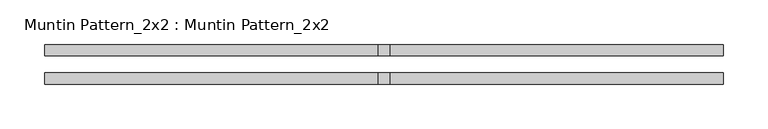
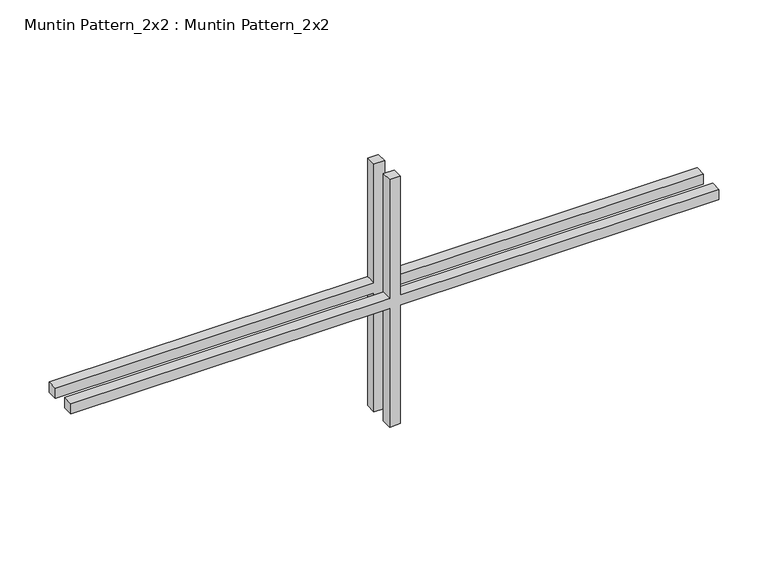
"""IFC4 building model written with IfcOpenShell, lengths in millimetres: proxy geometry, Muntin Pattern_2x2 : Muntin Pattern_2x2."""

from ifc_helpers import new_model, si_unit, frame, origin, place, context, project, spatial, polyline, outline, extrude, source, transform, mapped, element, save


def muntin_pattern_2x2_muntin_pattern_2x2_101ea2c0(model_context):
    return source(origin(), model_context, "Body", "SweptSolid", [
        extrude(outline(polyline([(160.3375, -6.35), (160.3375, -381.0), (147.6375, -381.0), (147.6375, -6.35), (0.0, -6.35), (0.0, 6.35), (147.6375, 6.35), (147.6375, 381.0), (160.3375, 381.0), (160.3375, 6.35), (307.975, 6.35), (307.975, -6.35), (160.3375, -6.35)])), frame((0.0, 9.525, 0.0), z_axis=(0.0, 1.0, 0.0), x_axis=(0.0, 0.0, 1.0)), (0.0, 0.0, 1.0), 12.7),
        extrude(outline(polyline([(160.3375, -6.35), (160.3375, -381.0), (147.6375, -381.0), (147.6375, -6.35), (0.0, -6.35), (0.0, 6.35), (147.6375, 6.35), (147.6375, 381.0), (160.3375, 381.0), (160.3375, 6.35), (307.975, 6.35), (307.975, -6.35), (160.3375, -6.35)])), frame((0.0, -22.225, 0.0), z_axis=(0.0, 1.0, 0.0), x_axis=(0.0, 0.0, 1.0)), (0.0, 0.0, 1.0), 12.7),
    ])


if __name__ == "__main__":
    model = new_model("IFC4")
    model_context = context("Model", 3, world=origin())
    ifc_project = project(units=[si_unit("LENGTHUNIT", "METRE", prefix="MILLI")], contexts=[model_context])
    site = spatial("IfcSite", under=ifc_project)
    building = spatial("IfcBuilding", under=site)
    placement = place(None, origin())
    muntin_pattern_2x2_muntin_pattern_2x2_shape = muntin_pattern_2x2_muntin_pattern_2x2_101ea2c0(model_context)
    element("IfcBuildingElementProxy", 1, Name="Muntin Pattern_2x2 : Muntin Pattern_2x2", ObjectType="Muntin Pattern_2x2 : Muntin Pattern_2x2", at=placement, inside=building, context=model_context, shape_type="MappedRepresentation", body=[
        mapped(muntin_pattern_2x2_muntin_pattern_2x2_shape, transform((0.0, 0.0, 0.0), x_axis=(1.0, 0.0, 0.0), y_axis=(0.0, 1.0, 0.0), z_axis=(0.0, 0.0, 1.0))),
    ])
    save(model, "model.ifc")

# Revit data of these elements
# Type "Muntin Pattern_2x2 : Muntin Pattern_2x2"
#   Width [instance default] = 4' - 0"
#   Thickness = 0' - 0 1/2"
#   Height [instance default] = 4' - 0"
#   Distance = 0' - 0 3/4"
#   Interior Material [instance default] = none
#   Exterior Material [instance default] = none
#   Default Elevation = 0
# Element 1 (IfcBuildingElementProxy, "Muntin Pattern_2x2 : Muntin Pattern_2x2")
#   Width = 2' - 6"
#   Height = 1' - 0 1/8"
#   Interior Material = Maple - Semigloss(Rotated)
#   Exterior Material = Clad - White
#   Materials on its faces: "Clad - White", "Maple - Semigloss(Rotated)"
# Materials
#   "Clad - White": class "Wood", colour RGB 245 245 243, transparency 0, Cost = 0
#   "Maple - Semigloss(Rotated)": class "Wood", colour RGB 196 161 118, transparency 0, Description = "Acer Saccharum", Cost = 0
